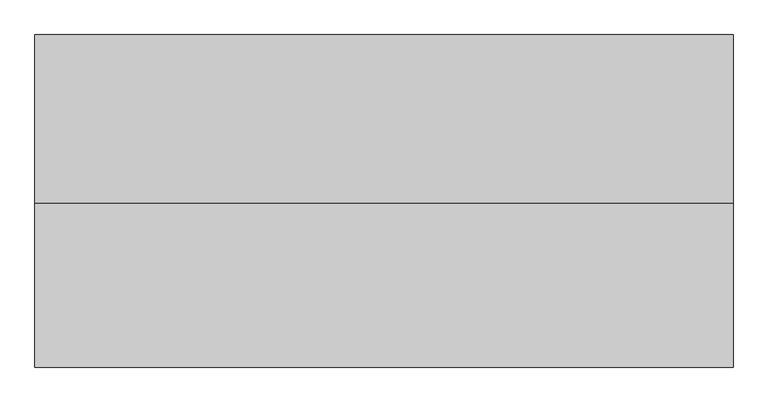
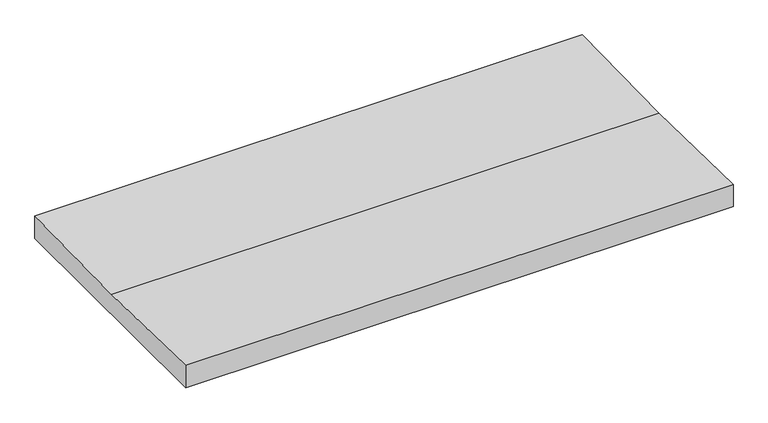
"""IFC4 building model written with IfcOpenShell, lengths in millimetres: proxy geometry, FIRESTONE INSULATION001 : FIRESTONE INSULATION001."""

from ifc_helpers import new_model, si_unit, frame, origin, place, context, project, spatial, polyline, outline, extrude, source, transform, mapped, element, save


def generic_models_30e3fc02(model_context):
    return source(origin(), model_context, "Body", "SweptSolid", [
        extrude(outline(polyline([(-4872.9612169, 40191.7185529), (-4390.315464, 40201.5164062), (-4390.315464, 40114.8623973), (-5343.2581759, 40114.8623973), (-5343.2581759, 40201.5164062), (-4872.9612169, 40191.7185529)])), frame((12382.7678845, 0.0, 0.0), z_axis=(1.0, 0.0, 0.0), x_axis=(0.0, 1.0, 0.0)), (0.0, 0.0, 1.0), 2000.25),
    ])


if __name__ == "__main__":
    model = new_model("IFC4")
    model_context = context("Model", 3, world=origin())
    ifc_project = project(units=[si_unit("LENGTHUNIT", "METRE", prefix="MILLI")], contexts=[model_context])
    site = spatial("IfcSite", under=ifc_project)
    building = spatial("IfcBuilding", under=site)
    placement = place(None, origin())
    generic_models_shape = generic_models_30e3fc02(model_context)
    element("IfcBuildingElementProxy", 1, Name="FIRESTONE INSULATION001 : FIRESTONE INSULATION001", ObjectType="FIRESTONE INSULATION001 : FIRESTONE INSULATION001", at=placement, inside=building, context=model_context, shape_type="MappedRepresentation", body=[
        mapped(generic_models_shape, transform((0.0, 0.0, 0.0), x_axis=(1.0, 0.0, 0.0), y_axis=(0.0, 1.0, 0.0), z_axis=(0.0, 0.0, 1.0))),
    ])
    save(model, "model.ifc")

# Revit data of these elements
# Type "FIRESTONE INSULATION001 : FIRESTONE INSULATION001"
#   NameOverride = "FIRESTONE INSULATION001"
# Element 1 (IfcBuildingElementProxy, "FIRESTONE INSULATION001 : FIRESTONE INSULATION001")
#   Materials on its faces: "TAPERED 2X SLEEPERS - SLOPED TO DRAIN"
# Materials
#   "TAPERED 2X SLEEPERS - SLOPED TO DRAIN": class "Unassigned", colour RGB 234 198 178, transparency 0
